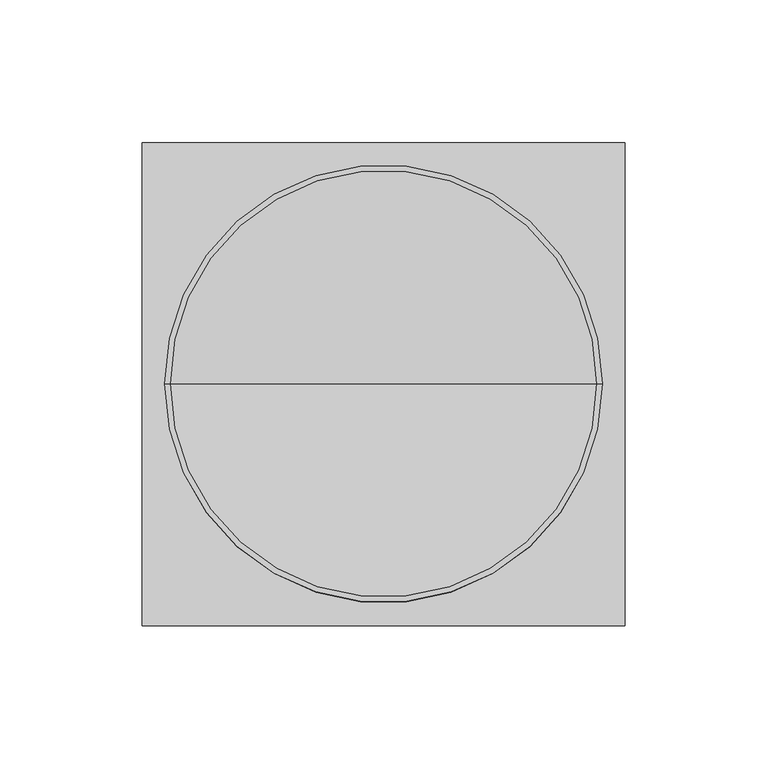
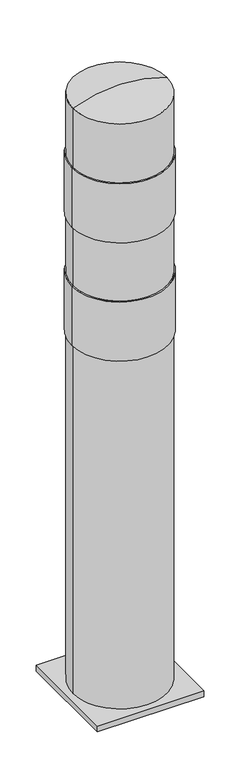
"""IFC4 building model written with IfcOpenShell, lengths in millimetres: proxy geometry, Signage_All_Loading-Systems_Safety-Bollardsrfa : H_GM_AR_B07_Steel Bollard_D150."""

import ifcopenshell
import ifcopenshell.guid

model = None  # the IFC model being written
_history = None  # IfcOwnerHistory: only IFC2X3 demands one
_inside = {}  # id of a spatial element -> (the spatial element, [elements in it])
_under = {}  # id of a project, library or spatial element -> (it, [spatial elements below it])
_declared = {}  # id of a project -> (the project, [libraries it declares])
_typed = {}  # id of a type object -> (the type object, [elements of that type])
_made_of = {}  # id of a material, layer set ... -> (it, [elements and type objects made of it])


def new_model(schema):
    """Start an empty IFC model of exactly this schema.

    Asked for "IFC4X3", IfcOpenShell would pick the latest addendum, in which some entities
    have other attributes; the version numbers below select the first issue.
    IFC2X3 requires an IfcOwnerHistory on every rooted entity: one is made here for all.
    """
    global model, _history
    if schema == "IFC4X3":
        model = ifcopenshell.file(schema_version=(4, 3, 0, 0))
    else:
        model = ifcopenshell.file(schema=schema)
    _inside.clear()
    _under.clear()
    _declared.clear()
    _typed.clear()
    _made_of.clear()
    _history = None
    if model.schema == "IFC2X3":
        org = make("IfcOrganization", Name="unknown")
        user = make(
            "IfcPersonAndOrganization",
            ThePerson=make("IfcPerson", FamilyName="unknown"),
            TheOrganization=org,
        )
        app = make(
            "IfcApplication",
            ApplicationDeveloper=org,
            Version="unknown",
            ApplicationFullName="unknown",
            ApplicationIdentifier="unknown",
        )
        _history = make(
            "IfcOwnerHistory",
            OwningUser=user,
            OwningApplication=app,
            ChangeAction="ADDED",
            CreationDate=0,
        )
    return model


def make(cls, **values):
    """One entity of the class cls with the attributes given. An attribute that is None is left unset."""
    return model.create_entity(
        cls, **{name: value for name, value in values.items() if value is not None}
    )


def rooted(cls, **values):
    """An entity with a GlobalId (a new one), such as an element, a storey or a relation."""
    return make(cls, GlobalId=ifcopenshell.guid.new(), OwnerHistory=_history, **values)


def si_unit(unit_type, name, prefix=None):
    """IfcSIUnit, for example si_unit("LENGTHUNIT", "METRE", prefix="MILLI")."""
    return make("IfcSIUnit", UnitType=unit_type, Prefix=prefix, Name=name)


def assignment(units):
    """IfcUnitAssignment: the units of a project."""
    return None if units is None else make("IfcUnitAssignment", Units=units)


def point(xyz):
    """IfcCartesianPoint."""
    return None if xyz is None else make("IfcCartesianPoint", Coordinates=xyz)


def direction(xyz):
    """IfcDirection."""
    return None if xyz is None else make("IfcDirection", DirectionRatios=xyz)


def frame(location, z_axis=None, x_axis=None):
    """IfcAxis2Placement3D, a coordinate frame: its origin and axes. An axis left out is left unset."""
    return make(
        "IfcAxis2Placement3D",
        Location=point(location),
        Axis=direction(z_axis),
        RefDirection=direction(x_axis),
    )


def origin():
    """The frame at (0, 0, 0) with its axes left unset."""
    return frame((0.0, 0.0, 0.0))


def origin_with_axes():
    """The frame at (0, 0, 0) with the z axis (0, 0, 1) and the x axis (1, 0, 0) written out."""
    return frame((0.0, 0.0, 0.0), z_axis=(0.0, 0.0, 1.0), x_axis=(1.0, 0.0, 0.0))


def place(relative_to, where):
    """IfcLocalPlacement: puts the frame where relative to a parent placement (None: the world)."""
    return make(
        "IfcLocalPlacement", PlacementRelTo=relative_to, RelativePlacement=where
    )


def context(
    kind, dimensions, precision=None, world=None, true_north=None, identifier=None
):
    """IfcGeometricRepresentationContext, for example the 3D "Model" context."""
    return make(
        "IfcGeometricRepresentationContext",
        ContextIdentifier=identifier,
        ContextType=kind,
        CoordinateSpaceDimension=dimensions,
        Precision=precision,
        WorldCoordinateSystem=world,
        TrueNorth=true_north,
    )


def project(units=None, contexts=None):
    """IfcProject with its units and contexts."""
    return rooted(
        "IfcProject",
        Name="project",
        RepresentationContexts=contexts,
        UnitsInContext=assignment(units),
    )


def spatial(cls, under=None, at=None, **own):
    """A site, building, storey or space (cls), placed at a placement, below another one or the project."""
    s = rooted(cls, ObjectPlacement=at, **own)
    if under is not None:
        _under.setdefault(under.id(), (under, []))[1].append(s)
    return s


def polyline(points):
    """IfcPolyline through the points."""
    return make("IfcPolyline", Points=[point(p) for p in points])


def circle_curve(where, radius):
    """IfcCircle in the frame where."""
    return make("IfcCircle", Position=where, Radius=radius)


def ellipse_curve(where, semi_axis1, semi_axis2):
    """IfcEllipse in the frame where."""
    return make(
        "IfcEllipse", Position=where, SemiAxis1=semi_axis1, SemiAxis2=semi_axis2
    )


def trimmed(basis, trim1, trim2, sense, master):
    """IfcTrimmedCurve: the piece of a basis curve between two trims."""
    return make(
        "IfcTrimmedCurve",
        BasisCurve=basis,
        Trim1=trim1,
        Trim2=trim2,
        SenseAgreement=sense,
        MasterRepresentation=master,
    )


def outline(outer, holes=None, kind="AREA"):
    """IfcArbitraryClosedProfileDef: a profile drawn as a closed curve; with holes, ...WithVoids."""
    if holes is None:
        return make("IfcArbitraryClosedProfileDef", ProfileType=kind, OuterCurve=outer)
    return make(
        "IfcArbitraryProfileDefWithVoids",
        ProfileType=kind,
        OuterCurve=outer,
        InnerCurves=holes,
    )


def extrude(swept, where, along, depth):
    """IfcExtrudedAreaSolid: the profile swept, set in the frame where, extruded along a direction by depth."""
    return make(
        "IfcExtrudedAreaSolid",
        SweptArea=swept,
        Position=where,
        ExtrudedDirection=direction(along),
        Depth=depth,
    )


def shape(context_of_items, identifier, shape_type, items):
    """IfcShapeRepresentation: the items that make up one representation, for example the "Body"."""
    return make(
        "IfcShapeRepresentation",
        ContextOfItems=context_of_items,
        RepresentationIdentifier=identifier,
        RepresentationType=shape_type,
        Items=items,
    )


def source(mapping_origin, context_of_items, identifier, shape_type, items):
    """IfcRepresentationMap: a shape defined once, which mapped items show again and again."""
    return make(
        "IfcRepresentationMap",
        MappingOrigin=mapping_origin,
        MappedRepresentation=shape(context_of_items, identifier, shape_type, items),
    )


def transform(
    local_origin,
    x_axis=None,
    y_axis=None,
    z_axis=None,
    scale=None,
    scale2=None,
    scale3=None,
    uniform=True,
):
    """IfcCartesianTransformationOperator3D, or its non-uniform kind. x_axis, y_axis, z_axis: its Axis1, 2, 3."""
    if uniform:
        return make(
            "IfcCartesianTransformationOperator3D",
            Axis1=direction(x_axis),
            Axis2=direction(y_axis),
            LocalOrigin=point(local_origin),
            Scale=scale,
            Axis3=direction(z_axis),
        )
    return make(
        "IfcCartesianTransformationOperator3DnonUniform",
        Axis1=direction(x_axis),
        Axis2=direction(y_axis),
        LocalOrigin=point(local_origin),
        Scale=scale,
        Axis3=direction(z_axis),
        Scale2=scale2,
        Scale3=scale3,
    )


def mapped(mapping_source, mapping_target):
    """IfcMappedItem: shows the shape of a source again, moved by a transform."""
    return make(
        "IfcMappedItem", MappingSource=mapping_source, MappingTarget=mapping_target
    )


def made_of(thing, what):
    """Note that an element or type object is made of a material, layer set ...; save() writes the relation."""
    if what is not None:
        _made_of.setdefault(what.id(), (what, []))[1].append(thing)
    return thing


def element(
    cls,
    number,
    at=None,
    inside=None,
    cuts=None,
    type_object=None,
    material=None,
    context=None,
    identifier="Body",
    shape_type=None,
    held_by="IfcProductDefinitionShape",
    body=None,
    shapes=None,
    **own,
):
    """One element of the class cls, such as IfcWall. Its Tag is "e" and its number.

    at: its placement. inside: the storey or other place that contains it. cuts: it is an
    opening in that element (IfcRelVoidsElement). A single representation is given by context,
    identifier, shape_type and body (its items); several are given by shapes. held_by: the class
    of the entity that holds the representations. save() writes the other relations.
    """
    e = rooted(cls, Tag="e%d" % number, ObjectPlacement=at, **own)
    if body is not None:
        shapes = [shape(context, identifier, shape_type, body)]
    if shapes is not None:
        e.Representation = make(held_by, Representations=shapes)
    if inside is not None:
        _inside.setdefault(inside.id(), (inside, []))[1].append(e)
    if cuts is not None:
        rooted(
            "IfcRelVoidsElement", RelatingBuildingElement=cuts, RelatedOpeningElement=e
        )
    if type_object is not None:
        _typed.setdefault(type_object.id(), (type_object, []))[1].append(e)
    return made_of(e, material)


def aggregate(whole, parts):
    """IfcRelAggregates: a whole, such as a stair, and the parts it consists of."""
    return rooted("IfcRelAggregates", RelatingObject=whole, RelatedObjects=parts)


def save(model, path):
    """Write the relations noted so far, then the file.

    IfcRelAggregates (storeys below a building ...), IfcRelContainedInSpatialStructure (elements
    in a storey), IfcRelDefinesByType, IfcRelAssociatesMaterial and IfcRelDeclares: one each for
    every whole, place, type object, material and project.
    """
    for whole, parts in _under.values():
        aggregate(whole, parts)
    for where, things in _inside.values():
        rooted(
            "IfcRelContainedInSpatialStructure",
            RelatedElements=things,
            RelatingStructure=where,
        )
    for kind, things in _typed.values():
        rooted("IfcRelDefinesByType", RelatedObjects=things, RelatingType=kind)
    for what, things in _made_of.values():
        rooted("IfcRelAssociatesMaterial", RelatedObjects=things, RelatingMaterial=what)
    for by, libraries in _declared.values():
        rooted("IfcRelDeclares", RelatingContext=by, RelatedDefinitions=libraries)
    model.write(path)


def plane_surface(at):
    """IfcPlane: the flat surface through the origin of the frame at, square to its z axis."""
    return make("IfcPlane", Position=at)


def cylinder_surface(at, radius):
    """IfcCylindricalSurface: all points at the distance radius from the z axis of the frame at."""
    return make("IfcCylindricalSurface", Position=at, Radius=radius)


def revolved_surface(curve, axis_point, axis_direction):
    """IfcSurfaceOfRevolution: the curve turned about the line through axis_point along axis_direction."""
    return make(
        "IfcSurfaceOfRevolution",
        SweptCurve=make("IfcArbitraryOpenProfileDef", ProfileType="CURVE", Curve=curve),
        AxisPosition=make("IfcAxis1Placement", Location=point(axis_point), Axis=direction(axis_direction)),
    )


def advanced_brep(points, edges, surfaces, faces):
    """IfcAdvancedBrep: a solid bounded by faces that lie on surfaces and meet in shared edges.

    An edge is (start, end): straight between two places in points (the first is 0);
    or (start, end, curve); or (start, end, curve, False) where it runs against its curve.
    A face is (place in surfaces, loops), or (place, loops, False) where it looks against
    its surface's normal. A loop lists edges by number (the first is 1), with a minus sign
    where the edge is run from its end to its start. The first loop is the outer one.
    """
    corners = [point(p) for p in points]
    vertices = [make("IfcVertexPoint", VertexGeometry=c) for c in corners]
    made = []
    for start, end, *more in edges:
        made.append(
            make(
                "IfcEdgeCurve",
                EdgeStart=vertices[start],
                EdgeEnd=vertices[end],
                EdgeGeometry=more[0] if more else make("IfcPolyline", Points=[corners[start], corners[end]]),
                SameSense=more[1] if len(more) > 1 else True,
            )
        )
    hull = []
    for where, loops, *sense in faces:
        bounds = []
        for j, loop in enumerate(loops):
            ring = [make("IfcOrientedEdge", EdgeElement=made[abs(k) - 1], Orientation=k > 0) for k in loop]
            bounds.append(
                make(
                    "IfcFaceOuterBound" if j == 0 else "IfcFaceBound",
                    Bound=make("IfcEdgeLoop", EdgeList=ring),
                    Orientation=True,
                )
            )
        hull.append(make("IfcAdvancedFace", Bounds=bounds, FaceSurface=surfaces[where], SameSense=sense[0] if sense else True))
    return make("IfcAdvancedBrep", Outer=make("IfcClosedShell", CfsFaces=hull))


def generic_models_1bc9e902(model_context):
    return source(origin(), model_context, "Body", "SolidModel", [
        advanced_brep(
        [(-70.0942839, 0.0, 800.0), (-147.0942839, 0.0, 800.0), (6.9057161, 0.0, 800.0), (6.9057161, 0.0, 900.0), (-147.0942839, 0.0, 900.0), (-70.0942839, 0.0, 900.0)],
        [
            (0, 1),
            (1, 2, circle_curve(frame((-70.0942839, 0.0, 800.0), z_axis=(0.0, 0.0, -1.0), x_axis=(-1.0, 0.0, 0.0)), 77.0)),
            (2, 0),
            (2, 1, circle_curve(frame((-70.0942839, 0.0, 800.0), z_axis=(0.0, 0.0, -1.0), x_axis=(-1.0, 0.0, 0.0)), 77.0)),
            (3, 4, circle_curve(frame((-70.0942839, 0.0, 900.0), z_axis=(0.0, 0.0, 1.0), x_axis=(-1.0, 0.0, 0.0)), 77.0)),
            (4, 5),
            (5, 3),
            (4, 3, circle_curve(frame((-70.0942839, 0.0, 900.0), z_axis=(0.0, 0.0, 1.0), x_axis=(-1.0, 0.0, 0.0)), 77.0)),
            (1, 4),
            (3, 2),
        ],
        [
            plane_surface(frame((-70.0942839, 0.0, 800.0), z_axis=(0.0, 0.0, -1.0), x_axis=(-1.0, 0.0, 0.0))),
            plane_surface(frame((-70.0942839, 0.0, 900.0), z_axis=(0.0, 0.0, 1.0), x_axis=(-1.0, 0.0, 0.0))),
            cylinder_surface(frame((-70.0942839, 0.0, 1210.0), z_axis=(0.0, 0.0, -1.0), x_axis=(-1.0, 0.0, 0.0)), 77.0),
        ],
        [
            (0, [[1, 2, 3]]),
            (0, [[-3, 4, -1]]),
            (1, [[5, 6, 7]]),
            (1, [[8, -7, -6]]),
            (2, [[-2, 9, -5, 10]]),
            (2, [[-4, -10, -8, -9]]),
        ],
    ),
        advanced_brep(
        [(-70.0942839, 0.0, 600.0), (-147.0942839, 0.0, 600.0), (6.9057161, 0.0, 600.0), (6.9057161, 0.0, 700.0), (-147.0942839, 0.0, 700.0), (-70.0942839, 0.0, 700.0)],
        [
            (0, 1),
            (1, 2, circle_curve(frame((-70.0942839, 0.0, 600.0), z_axis=(0.0, 0.0, -1.0), x_axis=(-1.0, 0.0, 0.0)), 77.0)),
            (2, 0),
            (2, 1, circle_curve(frame((-70.0942839, 0.0, 600.0), z_axis=(0.0, 0.0, -1.0), x_axis=(-1.0, 0.0, 0.0)), 77.0)),
            (3, 4, circle_curve(frame((-70.0942839, 0.0, 700.0), z_axis=(0.0, 0.0, 1.0), x_axis=(-1.0, 0.0, 0.0)), 77.0)),
            (4, 5),
            (5, 3),
            (4, 3, circle_curve(frame((-70.0942839, 0.0, 700.0), z_axis=(0.0, 0.0, 1.0), x_axis=(-1.0, 0.0, 0.0)), 77.0)),
            (1, 4),
            (3, 2),
        ],
        [
            plane_surface(frame((-70.0942839, 0.0, 600.0), z_axis=(0.0, 0.0, -1.0), x_axis=(-1.0, 0.0, 0.0))),
            plane_surface(frame((-70.0942839, 0.0, 700.0), z_axis=(0.0, 0.0, 1.0), x_axis=(-1.0, 0.0, 0.0))),
            cylinder_surface(frame((-70.0942839, 0.0, 1210.0), z_axis=(0.0, 0.0, -1.0), x_axis=(-1.0, 0.0, 0.0)), 77.0),
        ],
        [
            (0, [[1, 2, 3]]),
            (0, [[-3, 4, -1]]),
            (1, [[5, 6, 7]]),
            (1, [[8, -7, -6]]),
            (2, [[-2, 9, -5, 10]]),
            (2, [[-4, -10, -8, -9]]),
        ],
    ),
        advanced_brep(
        [(4.9057161, 0.0, 600.0), (-145.0942839, 0.0, 600.0), (-70.0942839, 0.0, 600.0), (-70.0942839, 0.0, 10.0), (-145.0942839, 0.0, 10.0), (4.9057161, 0.0, 10.0)],
        [
            (0, 1, circle_curve(frame((-70.0942839, 0.0, 600.0), z_axis=(0.0, 0.0, 1.0), x_axis=(-1.0, 0.0, 0.0)), 75.0)),
            (1, 2),
            (2, 0),
            (1, 0, circle_curve(frame((-70.0942839, 0.0, 600.0), z_axis=(0.0, 0.0, 1.0), x_axis=(-1.0, 0.0, 0.0)), 75.0)),
            (3, 4),
            (4, 5, circle_curve(frame((-70.0942839, 0.0, 10.0), z_axis=(0.0, 0.0, -1.0), x_axis=(-1.0, 0.0, 0.0)), 75.0)),
            (5, 3),
            (5, 4, circle_curve(frame((-70.0942839, 0.0, 10.0), z_axis=(0.0, 0.0, -1.0), x_axis=(-1.0, 0.0, 0.0)), 75.0)),
            (4, 1),
            (0, 5),
        ],
        [
            plane_surface(frame((-70.0942839, 0.0, 600.0), z_axis=(0.0, 0.0, 1.0), x_axis=(-1.0, 0.0, 0.0))),
            plane_surface(frame((-70.0942839, 0.0, 10.0), z_axis=(0.0, 0.0, -1.0), x_axis=(-1.0, 0.0, 0.0))),
            cylinder_surface(frame((-70.0942839, 0.0, 1060.0), z_axis=(0.0, 0.0, -1.0), x_axis=(-1.0, 0.0, 0.0)), 75.0),
        ],
        [
            (0, [[1, 2, 3]]),
            (0, [[4, -3, -2]]),
            (1, [[5, 6, 7]]),
            (1, [[-7, 8, -5]]),
            (2, [[-6, 9, -1, 10]]),
            (2, [[-8, -10, -4, -9]]),
        ],
    ),
        advanced_brep(
        [(-70.0942839, 0.0, 700.0), (-145.0942839, 0.0, 700.0), (4.9057161, 0.0, 700.0), (-145.0942839, 0.0, 800.0), (4.9057161, 0.0, 800.0), (-70.0942839, 0.0, 800.0)],
        [
            (0, 1),
            (1, 2, circle_curve(frame((-70.0942839, 0.0, 700.0), z_axis=(0.0, 0.0, -1.0), x_axis=(-1.0, 0.0, 0.0)), 75.0)),
            (2, 0),
            (2, 1, circle_curve(frame((-70.0942839, 0.0, 700.0), z_axis=(0.0, 0.0, -1.0), x_axis=(-1.0, 0.0, 0.0)), 75.0)),
            (1, 3),
            (3, 4, circle_curve(frame((-70.0942839, 0.0, 800.0), z_axis=(0.0, 0.0, -1.0), x_axis=(-1.0, 0.0, 0.0)), 75.0)),
            (4, 2),
            (4, 3, circle_curve(frame((-70.0942839, 0.0, 800.0), z_axis=(0.0, 0.0, -1.0), x_axis=(-1.0, 0.0, 0.0)), 75.0)),
            (3, 5),
            (5, 4),
        ],
        [
            plane_surface(frame((-70.0942839, 0.0, 700.0), z_axis=(0.0, 0.0, -1.0), x_axis=(-1.0, 0.0, 0.0))),
            cylinder_surface(frame((-70.0942839, 0.0, 1060.0), z_axis=(0.0, 0.0, -1.0), x_axis=(-1.0, 0.0, 0.0)), 75.0),
            plane_surface(frame((-70.0942839, 0.0, 800.0), z_axis=(0.0, 0.0, 1.0), x_axis=(-1.0, 0.0, 0.0))),
        ],
        [
            (0, [[1, 2, 3]]),
            (0, [[-3, 4, -1]]),
            (1, [[-2, 5, 6, 7]]),
            (1, [[-4, -7, 8, -5]]),
            (2, [[-6, 9, 10]]),
            (2, [[-8, -10, -9]]),
        ],
    ),
        advanced_brep(
        [(4.9057161, 0.0, 1000.0), (-145.0942839, 0.0, 1000.0), (-70.0942839, 0.0, 1015.0), (-70.0942839, 0.0, 900.0), (-145.0942839, 0.0, 900.0), (4.9057161, 0.0, 900.0)],
        [
            (0, 1, circle_curve(frame((-70.0942839, 0.0, 1000.0), z_axis=(0.0, 0.0, 1.0), x_axis=(-1.0, 0.0, 0.0)), 75.0)),
            (1, 2, circle_curve(frame((-68.2073512, 0.0, 810.5653364), z_axis=(0.0, 1.0, 0.0), x_axis=(1.0, 0.0, 0.0)), 204.4433716)),
            (2, 0, circle_curve(frame((-71.9812166, 0.0, 810.5653364), z_axis=(0.0, 1.0, 0.0), x_axis=(-1.0, 0.0, 0.0)), 204.4433716)),
            (1, 0, circle_curve(frame((-70.0942839, 0.0, 1000.0), z_axis=(0.0, 0.0, 1.0), x_axis=(-1.0, 0.0, 0.0)), 75.0)),
            (3, 4),
            (4, 5, circle_curve(frame((-70.0942839, 0.0, 900.0), z_axis=(0.0, 0.0, -1.0), x_axis=(-1.0, 0.0, 0.0)), 75.0)),
            (5, 3),
            (5, 4, circle_curve(frame((-70.0942839, 0.0, 900.0), z_axis=(0.0, 0.0, -1.0), x_axis=(-1.0, 0.0, 0.0)), 75.0)),
            (4, 1),
            (0, 5),
        ],
        [
            revolved_surface(trimmed(ellipse_curve(frame((-68.2073512, 0.0, 810.5653364), z_axis=(0.0, -1.0, 0.0), x_axis=(1.0, 0.0, 0.0)), 204.4433716, 204.4433716), [point((-70.0942839, 0.0, 1015.0))], [point((-145.0942839, 0.0, 1000.0))], True, "CARTESIAN"), (-70.0942839, 0.0, 1060.0), (0.0, 0.0, -1.0)),
            plane_surface(frame((-70.0942839, 0.0, 900.0), z_axis=(0.0, 0.0, -1.0), x_axis=(-1.0, 0.0, 0.0))),
            cylinder_surface(frame((-70.0942839, 0.0, 1060.0), z_axis=(0.0, 0.0, -1.0), x_axis=(-1.0, 0.0, 0.0)), 75.0),
        ],
        [
            (0, [[1, 2, 3]]),
            (0, [[4, -3, -2]]),
            (1, [[5, 6, 7]]),
            (1, [[-7, 8, -5]]),
            (2, [[-6, 9, -1, 10]]),
            (2, [[-8, -10, -4, -9]]),
        ],
    ),
        extrude(outline(polyline([(14.9057161, 85.0), (14.9057161, -85.0), (-155.0942839, -85.0), (-155.0942839, 85.0), (14.9057161, 85.0)])), origin_with_axes(), (0.0, 0.0, 1.0), 10.0),
    ])


if __name__ == "__main__":
    model = new_model("IFC4")
    model_context = context("Model", 3, world=origin())
    ifc_project = project(units=[si_unit("LENGTHUNIT", "METRE", prefix="MILLI")], contexts=[model_context])
    site = spatial("IfcSite", under=ifc_project)
    building = spatial("IfcBuilding", under=site)
    placement = place(None, origin())
    generic_models_shape = generic_models_1bc9e902(model_context)
    element("IfcBuildingElementProxy", 1, Name="Signage_All_Loading-Systems_Safety-Bollardsrfa : H_GM_AR_B07_Steel Bollard_D150", ObjectType="Signage_All_Loading-Systems_Safety-Bollardsrfa : H_GM_AR_B07_Steel Bollard_D150", at=placement, inside=building, context=model_context, shape_type="MappedRepresentation", body=[
        mapped(generic_models_shape, transform((0.0, 0.0, 0.0), x_axis=(1.0, 0.0, 0.0), y_axis=(0.0, 1.0, 0.0), z_axis=(0.0, 0.0, 1.0))),
    ])
    save(model, "model.ifc")

# Revit data of these elements
# Type "Signage_All_Loading-Systems_Safety-Bollardsrfa : H_GM_AR_B07_Steel Bollard_D150"
#   UniFormat II Description = "Vehicular Equipment"
#   UniFormat II = "E1030"
#   UniClass 2.0 Description = "Stainless Steel Bollards"
#   UniClass 2.0 = "Pr_20_76_08_82"
#   UniClass 1.4 Description = "Bollards"
#   UniClass 1.4 = "L8111"
#   UNSPSC Description = "Fixed traffic bollard"
#   UNSPSC = "46161533"
#   NBS Reference Description = "Stainless steel bollards"
#   NBS Reference = "45-25-15/313"
#   MasterFormat 2014 Description = "Manufactured Metal Bollards"
#   MasterFormat 2014 = "32 39 13"
#   Keynote = "32 39 13"
#   IFC Category = "Ramp"
#   Copyright = "©2018 BIM Project s.r.o."
#   COBIe Category = ""
#   URL = "http://www.loading-systems.com/"
#   Type Comments = "The new robust Loading Systems safety bollards provide optimal protection around your loading and unloading area."
#   BIM Project Category = "Loading Equipment"
#   Model = "960-051"
#   Manufacturer = "LOADING SYSTEMS"
#   Description = "Safety bollards"
#   Assembly Code = "E1030300"
#   Weight = 10.00 kg
#   Top = 15 mm
#   Length = 170 mm
#   Height = 1000 mm
#   Diameter = 150 mm
#   Depth = 170 mm
#   Default Elevation = 0
# Element 1 (IfcBuildingElementProxy, "Signage_All_Loading-Systems_Safety-Bollardsrfa : H_GM_AR_B07_Steel Bollard_D150")
#   Materials on its faces: "Paint - Yellow", "Plastic - Loading Systems - Rubber - Black"
# Materials
#   "Paint - Yellow": class "Paint", colour RGB 255 255 0, transparency 0
#   "Plastic - Loading Systems - Rubber - Black": class "Plast", colour RGB 63 63 63, transparency 0, Cost = 0
